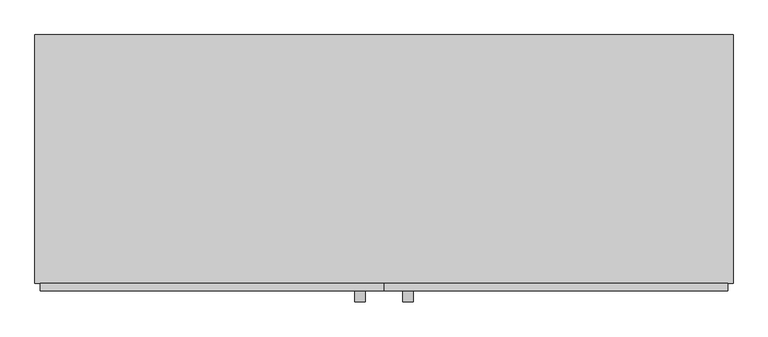
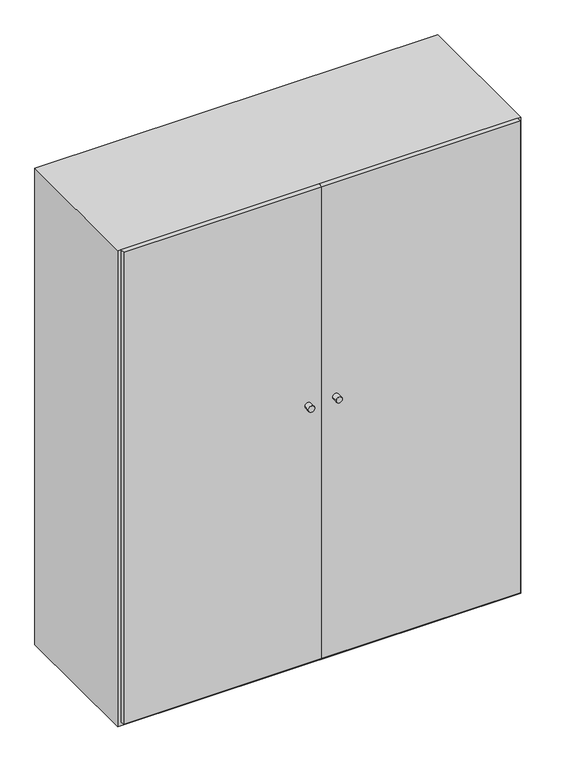
"""IFC4 building model written with IfcOpenShell, lengths in millimetres: furniture geometry, Armario dormitorio : ARMARIO DORM_PABLO."""

import ifcopenshell
import ifcopenshell.guid

model = None  # the IFC model being written
_history = None  # IfcOwnerHistory: only IFC2X3 demands one
_inside = {}  # id of a spatial element -> (the spatial element, [elements in it])
_under = {}  # id of a project, library or spatial element -> (it, [spatial elements below it])
_declared = {}  # id of a project -> (the project, [libraries it declares])
_typed = {}  # id of a type object -> (the type object, [elements of that type])
_made_of = {}  # id of a material, layer set ... -> (it, [elements and type objects made of it])


def new_model(schema):
    """Start an empty IFC model of exactly this schema.

    Asked for "IFC4X3", IfcOpenShell would pick the latest addendum, in which some entities
    have other attributes; the version numbers below select the first issue.
    IFC2X3 requires an IfcOwnerHistory on every rooted entity: one is made here for all.
    """
    global model, _history
    if schema == "IFC4X3":
        model = ifcopenshell.file(schema_version=(4, 3, 0, 0))
    else:
        model = ifcopenshell.file(schema=schema)
    _inside.clear()
    _under.clear()
    _declared.clear()
    _typed.clear()
    _made_of.clear()
    _history = None
    if model.schema == "IFC2X3":
        org = make("IfcOrganization", Name="unknown")
        user = make(
            "IfcPersonAndOrganization",
            ThePerson=make("IfcPerson", FamilyName="unknown"),
            TheOrganization=org,
        )
        app = make(
            "IfcApplication",
            ApplicationDeveloper=org,
            Version="unknown",
            ApplicationFullName="unknown",
            ApplicationIdentifier="unknown",
        )
        _history = make(
            "IfcOwnerHistory",
            OwningUser=user,
            OwningApplication=app,
            ChangeAction="ADDED",
            CreationDate=0,
        )
    return model


def make(cls, **values):
    """One entity of the class cls with the attributes given. An attribute that is None is left unset."""
    return model.create_entity(
        cls, **{name: value for name, value in values.items() if value is not None}
    )


def rooted(cls, **values):
    """An entity with a GlobalId (a new one), such as an element, a storey or a relation."""
    return make(cls, GlobalId=ifcopenshell.guid.new(), OwnerHistory=_history, **values)


def si_unit(unit_type, name, prefix=None):
    """IfcSIUnit, for example si_unit("LENGTHUNIT", "METRE", prefix="MILLI")."""
    return make("IfcSIUnit", UnitType=unit_type, Prefix=prefix, Name=name)


def assignment(units):
    """IfcUnitAssignment: the units of a project."""
    return None if units is None else make("IfcUnitAssignment", Units=units)


def point(xyz):
    """IfcCartesianPoint."""
    return None if xyz is None else make("IfcCartesianPoint", Coordinates=xyz)


def direction(xyz):
    """IfcDirection."""
    return None if xyz is None else make("IfcDirection", DirectionRatios=xyz)


def frame(location, z_axis=None, x_axis=None):
    """IfcAxis2Placement3D, a coordinate frame: its origin and axes. An axis left out is left unset."""
    return make(
        "IfcAxis2Placement3D",
        Location=point(location),
        Axis=direction(z_axis),
        RefDirection=direction(x_axis),
    )


def frame_2d(location, x_axis=None):
    """IfcAxis2Placement2D, a coordinate frame in the plane: its origin and x axis."""
    return make(
        "IfcAxis2Placement2D", Location=point(location), RefDirection=direction(x_axis)
    )


def origin():
    """The frame at (0, 0, 0) with its axes left unset."""
    return frame((0.0, 0.0, 0.0))


def origin_with_axes():
    """The frame at (0, 0, 0) with the z axis (0, 0, 1) and the x axis (1, 0, 0) written out."""
    return frame((0.0, 0.0, 0.0), z_axis=(0.0, 0.0, 1.0), x_axis=(1.0, 0.0, 0.0))


def place(relative_to, where):
    """IfcLocalPlacement: puts the frame where relative to a parent placement (None: the world)."""
    return make(
        "IfcLocalPlacement", PlacementRelTo=relative_to, RelativePlacement=where
    )


def context(
    kind, dimensions, precision=None, world=None, true_north=None, identifier=None
):
    """IfcGeometricRepresentationContext, for example the 3D "Model" context."""
    return make(
        "IfcGeometricRepresentationContext",
        ContextIdentifier=identifier,
        ContextType=kind,
        CoordinateSpaceDimension=dimensions,
        Precision=precision,
        WorldCoordinateSystem=world,
        TrueNorth=true_north,
    )


def project(units=None, contexts=None):
    """IfcProject with its units and contexts."""
    return rooted(
        "IfcProject",
        Name="project",
        RepresentationContexts=contexts,
        UnitsInContext=assignment(units),
    )


def spatial(cls, under=None, at=None, **own):
    """A site, building, storey or space (cls), placed at a placement, below another one or the project."""
    s = rooted(cls, ObjectPlacement=at, **own)
    if under is not None:
        _under.setdefault(under.id(), (under, []))[1].append(s)
    return s


def polyline(points):
    """IfcPolyline through the points."""
    return make("IfcPolyline", Points=[point(p) for p in points])


def circle_curve(where, radius):
    """IfcCircle in the frame where."""
    return make("IfcCircle", Position=where, Radius=radius)


def trimmed(basis, trim1, trim2, sense, master):
    """IfcTrimmedCurve: the piece of a basis curve between two trims."""
    return make(
        "IfcTrimmedCurve",
        BasisCurve=basis,
        Trim1=trim1,
        Trim2=trim2,
        SenseAgreement=sense,
        MasterRepresentation=master,
    )


def segment(curve, same_sense, transition):
    """IfcCompositeCurveSegment."""
    return make(
        "IfcCompositeCurveSegment",
        Transition=transition,
        SameSense=same_sense,
        ParentCurve=curve,
    )


def composite_curve(segments, self_intersect=None):
    """IfcCompositeCurve: segments joined end to end."""
    return make("IfcCompositeCurve", Segments=segments, SelfIntersect=self_intersect)


def outline(outer, holes=None, kind="AREA"):
    """IfcArbitraryClosedProfileDef: a profile drawn as a closed curve; with holes, ...WithVoids."""
    if holes is None:
        return make("IfcArbitraryClosedProfileDef", ProfileType=kind, OuterCurve=outer)
    return make(
        "IfcArbitraryProfileDefWithVoids",
        ProfileType=kind,
        OuterCurve=outer,
        InnerCurves=holes,
    )


def extrude(swept, where, along, depth):
    """IfcExtrudedAreaSolid: the profile swept, set in the frame where, extruded along a direction by depth."""
    return make(
        "IfcExtrudedAreaSolid",
        SweptArea=swept,
        Position=where,
        ExtrudedDirection=direction(along),
        Depth=depth,
    )


def shape(context_of_items, identifier, shape_type, items):
    """IfcShapeRepresentation: the items that make up one representation, for example the "Body"."""
    return make(
        "IfcShapeRepresentation",
        ContextOfItems=context_of_items,
        RepresentationIdentifier=identifier,
        RepresentationType=shape_type,
        Items=items,
    )


def source(mapping_origin, context_of_items, identifier, shape_type, items):
    """IfcRepresentationMap: a shape defined once, which mapped items show again and again."""
    return make(
        "IfcRepresentationMap",
        MappingOrigin=mapping_origin,
        MappedRepresentation=shape(context_of_items, identifier, shape_type, items),
    )


def transform(
    local_origin,
    x_axis=None,
    y_axis=None,
    z_axis=None,
    scale=None,
    scale2=None,
    scale3=None,
    uniform=True,
):
    """IfcCartesianTransformationOperator3D, or its non-uniform kind. x_axis, y_axis, z_axis: its Axis1, 2, 3."""
    if uniform:
        return make(
            "IfcCartesianTransformationOperator3D",
            Axis1=direction(x_axis),
            Axis2=direction(y_axis),
            LocalOrigin=point(local_origin),
            Scale=scale,
            Axis3=direction(z_axis),
        )
    return make(
        "IfcCartesianTransformationOperator3DnonUniform",
        Axis1=direction(x_axis),
        Axis2=direction(y_axis),
        LocalOrigin=point(local_origin),
        Scale=scale,
        Axis3=direction(z_axis),
        Scale2=scale2,
        Scale3=scale3,
    )


def mapped(mapping_source, mapping_target):
    """IfcMappedItem: shows the shape of a source again, moved by a transform."""
    return make(
        "IfcMappedItem", MappingSource=mapping_source, MappingTarget=mapping_target
    )


def made_of(thing, what):
    """Note that an element or type object is made of a material, layer set ...; save() writes the relation."""
    if what is not None:
        _made_of.setdefault(what.id(), (what, []))[1].append(thing)
    return thing


def element(
    cls,
    number,
    at=None,
    inside=None,
    cuts=None,
    type_object=None,
    material=None,
    context=None,
    identifier="Body",
    shape_type=None,
    held_by="IfcProductDefinitionShape",
    body=None,
    shapes=None,
    **own,
):
    """One element of the class cls, such as IfcWall. Its Tag is "e" and its number.

    at: its placement. inside: the storey or other place that contains it. cuts: it is an
    opening in that element (IfcRelVoidsElement). A single representation is given by context,
    identifier, shape_type and body (its items); several are given by shapes. held_by: the class
    of the entity that holds the representations. save() writes the other relations.
    """
    e = rooted(cls, Tag="e%d" % number, ObjectPlacement=at, **own)
    if body is not None:
        shapes = [shape(context, identifier, shape_type, body)]
    if shapes is not None:
        e.Representation = make(held_by, Representations=shapes)
    if inside is not None:
        _inside.setdefault(inside.id(), (inside, []))[1].append(e)
    if cuts is not None:
        rooted(
            "IfcRelVoidsElement", RelatingBuildingElement=cuts, RelatedOpeningElement=e
        )
    if type_object is not None:
        _typed.setdefault(type_object.id(), (type_object, []))[1].append(e)
    return made_of(e, material)


def aggregate(whole, parts):
    """IfcRelAggregates: a whole, such as a stair, and the parts it consists of."""
    return rooted("IfcRelAggregates", RelatingObject=whole, RelatedObjects=parts)


def save(model, path):
    """Write the relations noted so far, then the file.

    IfcRelAggregates (storeys below a building ...), IfcRelContainedInSpatialStructure (elements
    in a storey), IfcRelDefinesByType, IfcRelAssociatesMaterial and IfcRelDeclares: one each for
    every whole, place, type object, material and project.
    """
    for whole, parts in _under.values():
        aggregate(whole, parts)
    for where, things in _inside.values():
        rooted(
            "IfcRelContainedInSpatialStructure",
            RelatedElements=things,
            RelatingStructure=where,
        )
    for kind, things in _typed.values():
        rooted("IfcRelDefinesByType", RelatedObjects=things, RelatingType=kind)
    for what, things in _made_of.values():
        rooted("IfcRelAssociatesMaterial", RelatedObjects=things, RelatingMaterial=what)
    for by, libraries in _declared.values():
        rooted("IfcRelDeclares", RelatingContext=by, RelatedDefinitions=libraries)
    model.write(path)


def furniture_64353a5b(model_context):
    return source(origin(), model_context, "Body", "SweptSolid", [
        extrude(outline(composite_curve([segment(trimmed(circle_curve(frame_2d((1100.0, -55.0)), 12.5), [point((1100.0, -67.5))], [point((1100.0, -42.5))], False, "CARTESIAN"), True, "CONTINUOUS"), segment(trimmed(circle_curve(frame_2d((1100.0, -55.0)), 12.5), [point((1100.0, -42.5))], [point((1100.0, -67.5))], False, "CARTESIAN"), True, "CONTINUOUS")], self_intersect=False)), frame((0.0, -613.0, 0.0), z_axis=(0.0, 1.0, 0.0), x_axis=(0.0, 0.0, 1.0)), (0.0, 0.0, 1.0), 25.0),
        extrude(outline(composite_curve([segment(trimmed(circle_curve(frame_2d((1100.0, 55.0)), 12.5), [point((1100.0, 42.5))], [point((1100.0, 67.5))], False, "CARTESIAN"), True, "CONTINUOUS"), segment(trimmed(circle_curve(frame_2d((1100.0, 55.0)), 12.5), [point((1100.0, 67.5))], [point((1100.0, 42.5))], False, "CARTESIAN"), True, "CONTINUOUS")], self_intersect=False)), frame((0.0, -613.0, 0.0), z_axis=(0.0, 1.0, 0.0), x_axis=(0.0, 0.0, 1.0)), (0.0, 0.0, 1.0), 25.0),
        extrude(outline(polyline([(0.0, -570.0), (787.5, -570.0), (787.5, -588.0), (0.0, -588.0), (0.0, -570.0)])), frame((0.0, 0.0, 18.0), z_axis=(0.0, 0.0, 1.0), x_axis=(1.0, 0.0, 0.0)), (0.0, 0.0, 1.0), 1982.0),
        extrude(outline(polyline([(0.0, -570.0), (0.0, -588.0), (-787.5, -588.0), (-787.5, -570.0), (0.0, -570.0)])), frame((0.0, 0.0, 18.0), z_axis=(0.0, 0.0, 1.0), x_axis=(1.0, 0.0, 0.0)), (0.0, 0.0, 1.0), 1982.0),
        extrude(outline(polyline([(800.0, 0.0), (800.0, -570.0), (-800.0, -570.0), (-800.0, 0.0), (800.0, 0.0)])), origin_with_axes(), (0.0, 0.0, 1.0), 2000.0),
    ])


if __name__ == "__main__":
    model = new_model("IFC4")
    model_context = context("Model", 3, world=origin())
    ifc_project = project(units=[si_unit("LENGTHUNIT", "METRE", prefix="MILLI")], contexts=[model_context])
    site = spatial("IfcSite", under=ifc_project)
    building = spatial("IfcBuilding", under=site)
    placement = place(None, origin())
    furniture_shape = furniture_64353a5b(model_context)
    element("IfcFurniture", 1, ObjectType="Armario dormitorio : ARMARIO DORM_PABLO", at=placement, inside=building, context=model_context, shape_type="MappedRepresentation", body=[
        mapped(furniture_shape, transform((0.0, 0.0, 0.0), x_axis=(1.0, 0.0, 0.0), y_axis=(0.0, 1.0, 0.0), z_axis=(0.0, 0.0, 1.0))),
    ])
    save(model, "model.ifc")

# Revit data of these elements
# Type "Armario dormitorio : ARMARIO DORM_PABLO"
#   Anchura = 1.60 m
#   Altura = 2.00 m
#   Profundidad = 0.57 m
#   Material de armario = none
#   Default Elevation = 0
# Element 1 (IfcFurniture, "Armario dormitorio : ARMARIO DORM_PABLO")
#   Materials on its faces: "Madera - Listel"
# Materials
#   "Madera - Listel": class "Madera", colour RGB 210 180 110, transparency 0, Cost = 0
